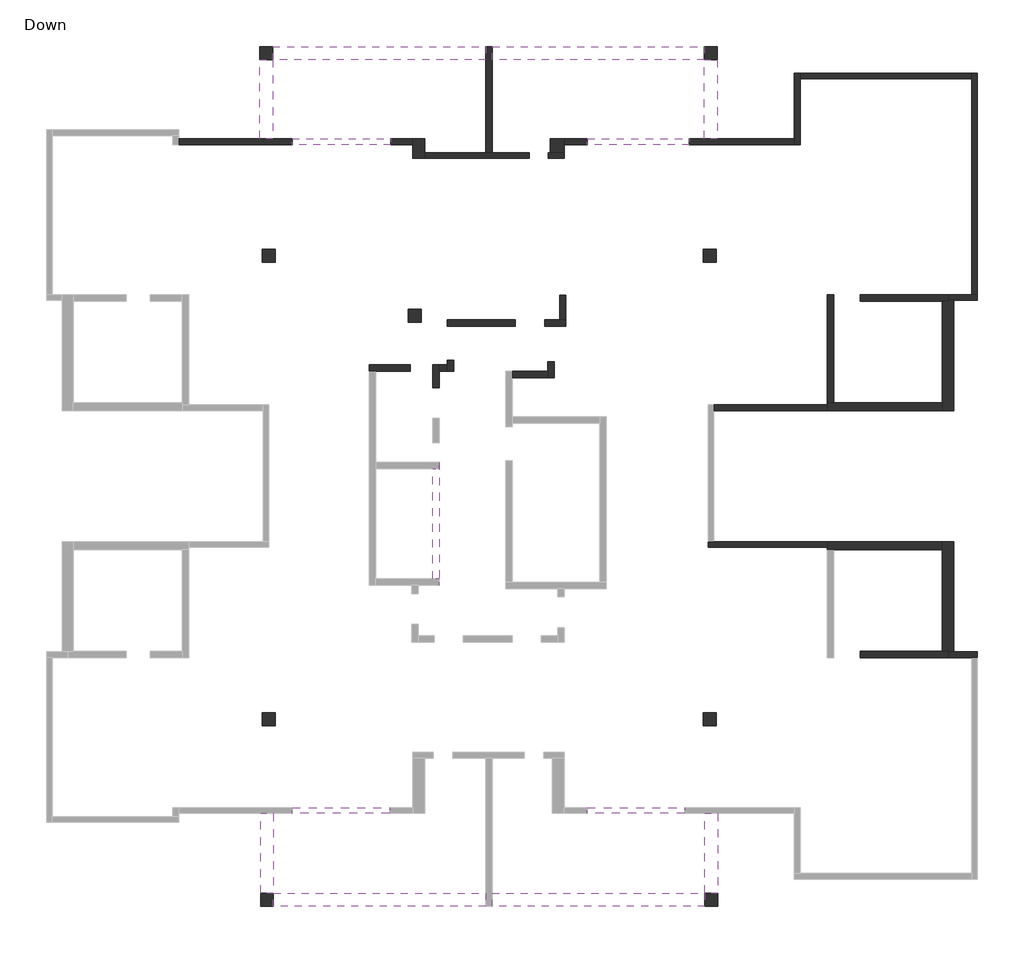
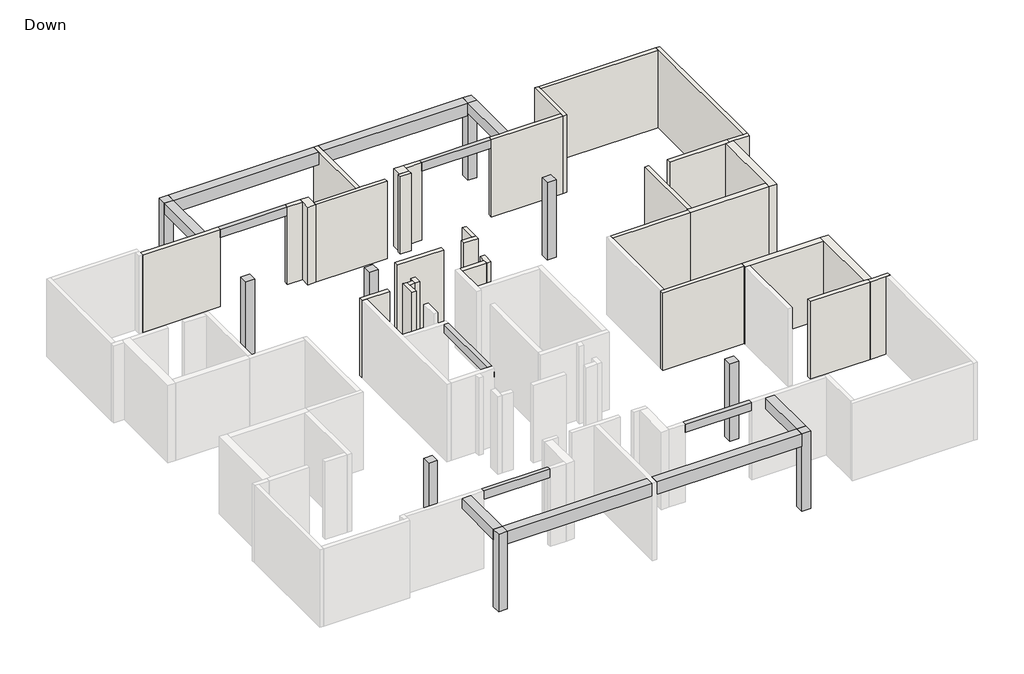
# One storey, part 2 of 2: 32 walls, 13 beams, 9 columns.
"""IFC4 building model written with IfcOpenShell, lengths in millimetres."""

from ifc_helpers import new_model, si_unit, origin, origin_with_axes, place, context, project, spatial, polyline, outline, extrude, faceted_brep, element, save

model = new_model("IFC4")

# Units and contexts
model_context = context("Model", 3, world=origin())
ifc_project = project(units=[si_unit("LENGTHUNIT", "METRE", prefix="MILLI")], contexts=[model_context])

# Site, building, storey
site = spatial("IfcSite", under=ifc_project)
building = spatial("IfcBuilding", under=site)
storey = spatial("IfcBuildingStorey", under=building, Name="Down", Elevation=0.0)

# Beams
placement = place(None, origin())
element("IfcBeam", 1, ObjectType="Concrete Rectengular Beam : 18/40", at=placement, inside=storey, context=model_context, shape_type="Brep", body=[
    faceted_brep([(-17031.2403988, 23917.8919264, 3700.0), (-17031.2403988, 23737.8919264, 3700.0), (-17031.2403988, 23737.8919264, 3540.0), (-17031.2403988, 23737.8919264, 3300.0), (-17031.2403988, 23917.8919264, 3300.0), (-17031.2403988, 23917.8919264, 3540.0), (-20181.0054246, 23917.8919264, 3300.0), (-20181.0054246, 23737.8919264, 3300.0), (-20181.0054246, 23737.8919264, 3540.0), (-20181.0054246, 23737.8919264, 3700.0), (-20181.0054246, 23917.8919264, 3700.0), (-20181.0054246, 23917.8919264, 3540.0)], [[[0, 1, 2, 3, 4, 5]], [[6, 7, 8, 9, 10, 11]], [[1, 0, 10, 9]], [[1, 9, 8, 7, 3, 2]], [[4, 3, 7, 6]], [[10, 0, 5, 4, 6, 11]]]),
])
element("IfcBeam", 2, ObjectType="Concrete Rectengular Beam : 18/40", at=placement, inside=storey, context=model_context, shape_type="Brep", body=[
    faceted_brep([(-29280.7432632, 23917.9715458, 3300.0), (-29280.7432632, 23737.9715458, 3300.0), (-29280.7432632, 23737.9715458, 3540.0), (-29280.7432632, 23737.9715458, 3700.0), (-29280.7432632, 23917.9715458, 3700.0), (-29280.7432632, 23917.9715458, 3540.0), (-26241.1471859, 23737.9715458, 3700.0), (-26241.1471859, 23917.9715458, 3700.0), (-26241.1471859, 23737.9715458, 3300.0), (-26241.1471859, 23917.9715458, 3300.0)], [[[0, 1, 2, 3, 4, 5]], [[4, 3, 6, 7]], [[2, 1, 8, 6, 3]], [[1, 0, 9, 8]], [[5, 4, 7, 9, 0]], [[7, 6, 8, 9]]]),
])
element("IfcBeam", 3, ObjectType="Concrete Rectengular Beam : 18/40", at=placement, inside=storey, context=model_context, shape_type="Brep", body=[
    faceted_brep([(-26281.3646827, 3296.899597, 3700.0), (-26281.3646827, 3116.899597, 3700.0), (-26281.3646827, 3116.899597, 3540.0), (-26281.3646827, 3116.899597, 3300.0), (-26281.3646827, 3296.899597, 3300.0), (-26281.3646827, 3296.899597, 3540.0), (-29280.7432632, 3296.899597, 3300.0), (-29280.7432632, 3116.899597, 3300.0), (-29280.7432632, 3116.899597, 3540.0), (-29280.7432632, 3116.899597, 3700.0), (-29280.7432632, 3296.899597, 3700.0), (-29280.7432632, 3296.899597, 3540.0)], [[[0, 1, 2, 3, 4, 5]], [[6, 7, 8, 9, 10, 11]], [[1, 0, 10, 9]], [[1, 9, 8, 7, 3, 2]], [[4, 3, 7, 6]], [[10, 0, 5, 4, 6, 11]]]),
])
element("IfcBeam", 4, ObjectType="Concrete Rectengular Beam : 18/40", at=placement, inside=storey, context=model_context, shape_type="Brep", body=[
    faceted_brep([(-17179.5101337, 3296.899597, 3700.0), (-17179.5101337, 3116.899597, 3700.0), (-17179.5101337, 3116.899597, 3540.0), (-17179.5101337, 3116.899597, 3300.0), (-17179.5101337, 3296.899597, 3300.0), (-17179.5101337, 3296.899597, 3540.0), (-20181.0054246, 3296.899597, 3300.0), (-20181.0054246, 3116.899597, 3300.0), (-20181.0054246, 3116.899597, 3540.0), (-20181.0054246, 3116.899597, 3700.0), (-20181.0054246, 3296.899597, 3700.0), (-20181.0054246, 3296.899597, 3540.0)], [[[0, 1, 2, 3, 4, 5]], [[6, 7, 8, 9, 10, 11]], [[1, 0, 10, 9]], [[1, 9, 8, 7, 3, 2]], [[4, 3, 7, 6]], [[10, 0, 5, 4, 6, 11]]]),
])
element("IfcBeam", 5, ObjectType="Concrete Rectengular Beam : 20/40", at=placement, inside=storey, context=model_context, shape_type="Brep", body=[
    faceted_brep([(-24949.9538662, 10346.5743227, 3700.0), (-24750.9830923, 10346.5743227, 3700.0), (-24750.9830923, 13748.1861297, 3700.0), (-24949.9538662, 13748.1861297, 3700.0), (-24949.9538662, 10346.5743227, 3300.0), (-24949.9538662, 13748.1861297, 3300.0), (-24749.9538662, 13948.1861297, 3300.0), (-24749.9538662, 10146.5743227, 3300.0), (-24750.9830923, 10146.5743227, 3300.0), (-24750.9830923, 10346.5743227, 3300.0), (-24750.9830923, 13748.1861297, 3300.0), (-24750.9830923, 13948.1861297, 3300.0), (-24749.9538662, 13948.1861297, 3540.0), (-24749.9538662, 10146.5743227, 3540.0), (-24750.9830923, 10146.5743227, 3540.0), (-24750.9830923, 13948.1861297, 3540.0), (-24750.9830923, 13748.1861297, 3540.0), (-24750.9830923, 10346.5743227, 3540.0)], [[[0, 1, 2, 3]], [[4, 0, 3, 5]], [[6, 7, 8, 9, 4, 5, 10, 11]], [[7, 6, 12, 13]], [[7, 13, 14, 8]], [[12, 6, 11, 15]], [[13, 12, 15, 16, 17, 14]], [[9, 17, 1, 0, 4]], [[17, 9, 8, 14]], [[16, 10, 5, 3, 2]], [[10, 16, 15, 11]], [[1, 17, 16, 2]]]),
])
element("IfcBeam", 6, ObjectType="Concrete Rectengular Beam : 40/50", at=placement, inside=storey, context=model_context, shape_type="Brep", body=[
    faceted_brep([(-29879.8305532, 26366.9840713, 3700.0), (-30279.8305532, 26366.9840713, 3700.0), (-30279.8305532, 23917.9715458, 3700.0), (-29879.8305532, 23917.9715458, 3700.0), (-29879.8305532, 26366.9840713, 3200.0), (-29879.8305532, 26366.9840713, 3540.0), (-29879.8305532, 23917.9715458, 3540.0), (-29879.8305532, 23917.9715458, 3200.0), (-30279.8305532, 26366.9840713, 3200.0), (-30279.8305532, 23917.9715458, 3200.0)], [[[0, 1, 2, 3]], [[4, 5, 0, 3, 6, 7]], [[8, 4, 7, 9]], [[1, 8, 9, 2]], [[1, 0, 5, 4, 8]], [[3, 2, 9, 7, 6]]]),
])
element("IfcBeam", 7, ObjectType="Concrete Rectengular Beam : 40/50", at=placement, inside=storey, context=model_context, shape_type="Brep", body=[
    faceted_brep([(-16180.4228437, 26366.9840713, 3700.0), (-16580.4228437, 26366.9840713, 3700.0), (-16580.4228437, 23917.8919264, 3700.0), (-16180.4228437, 23917.8919264, 3700.0), (-16180.4228437, 26366.9840713, 3200.0), (-16180.4228437, 23917.8919264, 3200.0), (-16580.4228437, 26366.9840713, 3200.0), (-16580.4228437, 23917.8919264, 3200.0), (-16580.4228437, 26366.9840713, 3540.0), (-16580.4228437, 23917.8919264, 3540.0)], [[[0, 1, 2, 3]], [[4, 0, 3, 5]], [[6, 4, 5, 7]], [[1, 8, 6, 7, 9, 2]], [[1, 0, 4, 6, 8]], [[3, 2, 9, 7, 5]]]),
])
element("IfcBeam", 8, ObjectType="Concrete Rectengular Beam : 40/50", at=placement, inside=storey, context=model_context, shape_type="Brep", body=[
    faceted_brep([(-30261.4923547, 659.7166846, 3700.0), (-29861.4923547, 659.7166846, 3700.0), (-29861.4923547, 3116.899597, 3700.0), (-30261.4923547, 3116.899597, 3700.0), (-29861.4923547, 659.7166846, 3540.0), (-29861.4923547, 659.7166846, 3200.0), (-29861.4923547, 3116.899597, 3200.0), (-29861.4923547, 3116.899597, 3540.0), (-30261.4923547, 659.7166846, 3200.0), (-30261.4923547, 3116.899597, 3200.0)], [[[0, 1, 2, 3]], [[1, 4, 5, 6, 7, 2]], [[5, 8, 9, 6]], [[8, 0, 3, 9]], [[5, 4, 1, 0, 8]], [[3, 2, 7, 6, 9]]]),
])
element("IfcBeam", 9, ObjectType="Concrete Rectengular Beam : 40/50", at=placement, inside=storey, context=model_context, shape_type="Brep", body=[
    faceted_brep([(-16561.2977307, 659.7166846, 3700.0), (-16161.2977307, 659.7166846, 3700.0), (-16161.2977307, 3116.899597, 3700.0), (-16561.2977307, 3116.899597, 3700.0), (-16561.2977307, 659.7166846, 3200.0), (-16561.2977307, 659.7166846, 3540.0), (-16561.2977307, 3116.899597, 3540.0), (-16561.2977307, 3116.899597, 3200.0), (-16161.2977307, 659.7166846, 3200.0), (-16161.2977307, 3116.899597, 3200.0)], [[[0, 1, 2, 3]], [[4, 5, 0, 3, 6, 7]], [[8, 4, 7, 9]], [[1, 8, 9, 2]], [[0, 5, 4, 8, 1]], [[3, 2, 9, 7, 6]]]),
])
element("IfcBeam", 10, ObjectType="Concrete Rectengular Beam : 40/60", at=placement, inside=storey, context=model_context, shape_type="Brep", body=[
    faceted_brep([(-29879.8305532, 26766.9840713, 3700.0), (-29879.8305532, 26366.9840713, 3700.0), (-23307.4000343, 26366.9840713, 3700.0), (-23307.4000343, 26766.9840713, 3700.0), (-29879.8305532, 26366.9840713, 3540.0), (-29879.8305532, 26366.9840713, 3100.0), (-23307.4000343, 26366.9840713, 3100.0), (-23307.4000343, 26366.9840713, 3540.0), (-29879.8305532, 26766.9840713, 3100.0), (-23307.4000343, 26766.9840713, 3100.0)], [[[0, 1, 2, 3]], [[1, 4, 5, 6, 7, 2]], [[5, 8, 9, 6]], [[8, 0, 3, 9]], [[1, 0, 8, 5, 4]], [[3, 2, 7, 6, 9]]]),
])
element("IfcBeam", 11, ObjectType="Concrete Rectengular Beam : 40/60", at=placement, inside=storey, context=model_context, shape_type="Brep", body=[
    faceted_brep([(-23107.4000343, 26766.9840713, 3700.0), (-23107.4000343, 26366.9840713, 3700.0), (-16580.4228437, 26366.9840713, 3700.0), (-16580.4228437, 26766.9840713, 3700.0), (-23107.4000343, 26366.9840713, 3540.0), (-23107.4000343, 26366.9840713, 3100.0), (-16580.4228437, 26366.9840713, 3100.0), (-16580.4228437, 26366.9840713, 3540.0), (-23107.4000343, 26766.9840713, 3100.0), (-16580.4228437, 26766.9840713, 3100.0)], [[[0, 1, 2, 3]], [[1, 4, 5, 6, 7, 2]], [[5, 8, 9, 6]], [[8, 0, 3, 9]], [[1, 0, 8, 5, 4]], [[3, 2, 7, 6, 9]]]),
])
element("IfcBeam", 12, ObjectType="Concrete Rectengular Beam : 40/60", at=placement, inside=storey, context=model_context, shape_type="Brep", body=[
    faceted_brep([(-29861.4923547, 659.7166846, 3700.0), (-29861.4923547, 259.7166846, 3700.0), (-23311.6200473, 259.7166846, 3700.0), (-23311.6200473, 659.7166846, 3700.0), (-29861.4923547, 259.7166846, 3100.0), (-23311.6200473, 259.7166846, 3100.0), (-29861.4923547, 659.7166846, 3100.0), (-23311.6200473, 659.7166846, 3100.0), (-29861.4923547, 659.7166846, 3540.0), (-23311.6200473, 659.7166846, 3540.0)], [[[0, 1, 2, 3]], [[1, 4, 5, 2]], [[4, 6, 7, 5]], [[6, 8, 0, 3, 9, 7]], [[1, 0, 8, 6, 4]], [[3, 2, 5, 7, 9]]]),
])
element("IfcBeam", 13, ObjectType="Concrete Rectengular Beam : 40/60", at=placement, inside=storey, context=model_context, shape_type="Brep", body=[
    faceted_brep([(-16561.2977307, 259.7166846, 3700.0), (-16561.2977307, 659.7166846, 3700.0), (-23111.6200473, 659.7166846, 3700.0), (-23111.6200473, 259.7166846, 3700.0), (-16561.2977307, 259.7166846, 3100.0), (-23111.6200473, 259.7166846, 3100.0), (-16561.2977307, 659.7166846, 3100.0), (-23111.6200473, 659.7166846, 3100.0), (-16561.2977307, 659.7166846, 3540.0), (-23111.6200473, 659.7166846, 3540.0)], [[[0, 1, 2, 3]], [[4, 0, 3, 5]], [[6, 4, 5, 7]], [[1, 8, 6, 7, 9, 2]], [[1, 0, 4, 6, 8]], [[3, 2, 9, 7, 5]]]),
])

# Columns
element("IfcColumn", 14, ObjectType="Concrete Rectengular Column : 40/40", at=placement, inside=storey, context=model_context, shape_type="Brep", body=[
    faceted_brep([(-16205.9170786, 20509.605542, 0.0), (-16205.9170786, 20109.605542, 0.0), (-16605.9170786, 20109.605542, 0.0), (-16605.9170786, 20509.605542, 0.0), (-16205.9170786, 20509.605542, 3700.0), (-16205.9170786, 20109.605542, 3700.0), (-16205.9170786, 20109.605542, 3540.0), (-16205.9170786, 20509.605542, 3540.0), (-16605.9170786, 20109.605542, 3700.0), (-16605.9170786, 20109.605542, 3540.0), (-16605.9170786, 20509.605542, 3700.0), (-16605.9170786, 20509.605542, 3540.0)], [[[0, 1, 2, 3]], [[4, 5, 6, 1, 0, 7]], [[5, 8, 9, 2, 1, 6]], [[8, 10, 11, 3, 2, 9]], [[10, 4, 7, 0, 3, 11]], [[4, 10, 8, 5]]]),
])
element("IfcColumn", 15, ObjectType="Concrete Rectengular Column : 40/40", at=placement, inside=storey, context=model_context, shape_type="Brep", body=[
    faceted_brep([(-29812.3773034, 20509.605542, 0.0), (-29812.3773034, 20109.605542, 0.0), (-30212.3773034, 20109.605542, 0.0), (-30212.3773034, 20509.605542, 0.0), (-29812.3773034, 20509.605542, 3700.0), (-29812.3773034, 20109.605542, 3700.0), (-29812.3773034, 20109.605542, 3540.0), (-29812.3773034, 20509.605542, 3540.0), (-30212.3773034, 20109.605542, 3700.0), (-30212.3773034, 20109.605542, 3540.0), (-30212.3773034, 20509.605542, 3700.0), (-30212.3773034, 20509.605542, 3540.0)], [[[0, 1, 2, 3]], [[4, 5, 6, 1, 0, 7]], [[5, 8, 9, 2, 1, 6]], [[8, 10, 11, 3, 2, 9]], [[10, 4, 7, 0, 3, 11]], [[4, 10, 8, 5]]]),
])
element("IfcColumn", 16, ObjectType="Concrete Rectengular Column : 40/40", at=placement, inside=storey, context=model_context, shape_type="Brep", body=[
    faceted_brep([(-29812.3773034, 6215.7849257, 0.0), (-29812.3773034, 5815.7849257, 0.0), (-30212.3773034, 5815.7849257, 0.0), (-30212.3773034, 6215.7849257, 0.0), (-29812.3773034, 6215.7849257, 3700.0), (-29812.3773034, 5815.7849257, 3700.0), (-29812.3773034, 5815.7849257, 3540.0), (-29812.3773034, 6215.7849257, 3540.0), (-30212.3773034, 5815.7849257, 3700.0), (-30212.3773034, 5815.7849257, 3540.0), (-30212.3773034, 6215.7849257, 3700.0), (-30212.3773034, 6215.7849257, 3540.0)], [[[0, 1, 2, 3]], [[4, 5, 6, 1, 0, 7]], [[5, 8, 9, 2, 1, 6]], [[8, 10, 11, 3, 2, 9]], [[10, 4, 7, 0, 3, 11]], [[4, 10, 8, 5]]]),
])
element("IfcColumn", 17, ObjectType="Concrete Rectengular Column : 40/40", at=placement, inside=storey, context=model_context, shape_type="Brep", body=[
    faceted_brep([(-16205.9170786, 6215.8431838, 0.0), (-16205.9170786, 5815.8431838, 0.0), (-16605.9170786, 5815.8431838, 0.0), (-16605.9170786, 6215.8431838, 0.0), (-16205.9170786, 6215.8431838, 3700.0), (-16205.9170786, 5815.8431838, 3700.0), (-16205.9170786, 5815.8431838, 3540.0), (-16205.9170786, 6215.8431838, 3540.0), (-16605.9170786, 5815.8431838, 3700.0), (-16605.9170786, 5815.8431838, 3540.0), (-16605.9170786, 6215.8431838, 3700.0), (-16605.9170786, 6215.8431838, 3540.0)], [[[0, 1, 2, 3]], [[4, 5, 6, 1, 0, 7]], [[5, 8, 9, 2, 1, 6]], [[8, 10, 11, 3, 2, 9]], [[10, 4, 7, 0, 3, 11]], [[4, 10, 8, 5]]]),
])
element("IfcColumn", 18, ObjectType="Concrete Rectengular Column : 40/40", at=placement, inside=storey, context=model_context, shape_type="Brep", body=[
    faceted_brep([(-16180.4228437, 26766.9840713, 0.0), (-16180.4228437, 26366.9840713, 0.0), (-16580.4228437, 26366.9840713, 0.0), (-16580.4228437, 26766.9840713, 0.0), (-16180.4228437, 26766.9840713, 3700.0), (-16180.4228437, 26366.9840713, 3700.0), (-16580.4228437, 26366.9840713, 3700.0), (-16580.4228437, 26366.9840713, 3100.0), (-16580.4228437, 26766.9840713, 3700.0), (-16580.4228437, 26766.9840713, 3100.0)], [[[0, 1, 2, 3]], [[4, 5, 1, 0]], [[5, 6, 7, 2, 1]], [[6, 8, 9, 3, 2, 7]], [[8, 4, 0, 3, 9]], [[4, 8, 6, 5]]]),
])
element("IfcColumn", 19, ObjectType="Concrete Rectengular Column : 40/40", at=placement, inside=storey, context=model_context, shape_type="Brep", body=[
    faceted_brep([(-29879.8305532, 26766.9840713, 0.0), (-29879.8305532, 26366.9840713, 0.0), (-30279.8305532, 26366.9840713, 0.0), (-30279.8305532, 26766.9840713, 0.0), (-29879.8305532, 26766.9840713, 3700.0), (-29879.8305532, 26366.9840713, 3700.0), (-29879.8305532, 26366.9840713, 3100.0), (-29879.8305532, 26766.9840713, 3100.0), (-30279.8305532, 26366.9840713, 3700.0), (-30279.8305532, 26766.9840713, 3700.0)], [[[0, 1, 2, 3]], [[4, 5, 6, 1, 0, 7]], [[5, 8, 2, 1, 6]], [[8, 9, 3, 2]], [[9, 4, 7, 0, 3]], [[4, 9, 8, 5]]]),
])
element("IfcColumn", 20, ObjectType="Concrete Rectengular Column : 40/40", at=placement, inside=storey, context=model_context, shape_type="SweptSolid", body=[
    extrude(outline(polyline([(-29861.4923547, 659.7166846), (-29861.4923547, 259.7166846), (-30261.4923547, 259.7166846), (-30261.4923547, 659.7166846), (-29861.4923547, 659.7166846)])), origin_with_axes(), (0.0, 0.0, 1.0), 3700.0),
])
element("IfcColumn", 21, ObjectType="Concrete Rectengular Column : 40/40", at=placement, inside=storey, context=model_context, shape_type="SweptSolid", body=[
    extrude(outline(polyline([(-16161.2977307, 659.7166846), (-16161.2977307, 259.7166846), (-16561.2977307, 259.7166846), (-16561.2977307, 659.7166846), (-16161.2977307, 659.7166846)])), origin_with_axes(), (0.0, 0.0, 1.0), 3700.0),
])
element("IfcColumn", 22, ObjectType="Concrete Rectengular Column : 40/40", at=placement, inside=storey, context=model_context, shape_type="Brep", body=[
    faceted_brep([(-25309.8528855, 18668.3919749, 0.0), (-25309.8528855, 18268.3919749, 0.0), (-25709.8528855, 18268.3919749, 0.0), (-25709.8528855, 18668.3919749, 0.0), (-25309.8528855, 18668.3919749, 3700.0), (-25309.8528855, 18268.3919749, 3700.0), (-25309.8528855, 18268.3919749, 3540.0), (-25309.8528855, 18668.3919749, 3540.0), (-25709.8528855, 18268.3919749, 3700.0), (-25709.8528855, 18268.3919749, 3540.0), (-25709.8528855, 18668.3919749, 3700.0), (-25709.8528855, 18668.3919749, 3540.0)], [[[0, 1, 2, 3]], [[4, 5, 6, 1, 0, 7]], [[5, 8, 9, 2, 1, 6]], [[8, 10, 11, 3, 2, 9]], [[10, 4, 7, 0, 3, 11]], [[4, 10, 8, 5]]]),
])

# Walls
element("IfcWall", 23, ObjectType="18", at=placement, inside=storey, context=model_context, shape_type="Brep", body=[
    faceted_brep([(-8149.623737, 8097.598694, 0.0), (-8879.8888113, 8097.598694, 0.0), (-9054.8888113, 8097.598694, 0.0), (-9054.8888113, 8097.598694, 3700.0), (-8879.8888113, 8097.598694, 3700.0), (-8149.623737, 8097.598694, 3700.0), (-8149.623737, 7917.598694, 0.0), (-8149.623737, 7917.598694, 3700.0), (-8329.623737, 7917.598694, 3700.0), (-9054.8888113, 7917.598694, 3700.0), (-9054.8888113, 7917.598694, 3540.0), (-9054.8888113, 7917.598694, 0.0), (-8329.623737, 7917.598694, 0.0)], [[[0, 1, 2, 3, 4, 5]], [[6, 7, 8, 9, 10, 11, 12]], [[2, 1, 0, 6, 12, 11]], [[3, 2, 11, 10, 9]], [[5, 4, 3, 9, 8, 7]], [[0, 5, 7, 6]]]),
])
element("IfcWall", 24, ObjectType="18", at=placement, inside=storey, context=model_context, shape_type="Brep", body=[
    faceted_brep([(-12779.898521, 11497.0355326, 0.0), (-16279.8286113, 11497.0355326, 0.0), (-16459.8286113, 11497.0355326, 0.0), (-16459.8286113, 11497.0355326, 3700.0), (-16279.8286113, 11497.0355326, 3700.0), (-12779.898521, 11497.0355326, 3700.0), (-12779.898521, 11317.0355326, 0.0), (-12779.898521, 11317.0355326, 3540.0), (-12779.898521, 11317.0355326, 3700.0), (-16459.8286113, 11317.0355326, 3700.0), (-16459.8286113, 11317.0355326, 3540.0), (-16459.8286113, 11317.0355326, 0.0)], [[[0, 1, 2, 3, 4, 5]], [[6, 7, 8, 9, 10, 11]], [[2, 1, 0, 6, 11]], [[5, 4, 3, 9, 8]], [[0, 5, 8, 7, 6]], [[3, 2, 11, 10, 9]]]),
])
element("IfcWall", 25, ObjectType="18", at=placement, inside=storey, context=model_context, shape_type="Brep", body=[
    faceted_brep([(-32781.782199, 23737.9715458, 0.0), (-29280.7432632, 23737.9715458, 0.0), (-29280.7432632, 23737.9715458, 3300.0), (-29280.7432632, 23737.9715458, 3700.0), (-32781.782199, 23737.9715458, 3700.0), (-32781.782199, 23917.9715458, 0.0), (-32781.782199, 23917.9715458, 3700.0), (-30279.8305532, 23917.9715458, 3700.0), (-29879.8305532, 23917.9715458, 3700.0), (-29280.7432632, 23917.9715458, 3700.0), (-29280.7432632, 23917.9715458, 3300.0), (-29280.7432632, 23917.9715458, 0.0)], [[[0, 1, 2, 3, 4]], [[5, 6, 7, 8, 9, 10, 11]], [[1, 0, 5, 11]], [[3, 2, 1, 11, 10, 9]], [[4, 3, 9, 8, 7, 6]], [[0, 4, 6, 5]]]),
])
element("IfcWall", 26, ObjectType="18", at=placement, inside=storey, context=model_context, shape_type="Brep", body=[
    faceted_brep([(-25199.7256887, 23316.7461841, 0.0), (-21979.7256887, 23316.7461841, 0.0), (-21979.7256887, 23316.7461841, 3700.0), (-25199.7256887, 23316.7461841, 3700.0), (-25199.7256887, 23496.7461841, 0.0), (-25199.7256887, 23496.7461841, 3540.0), (-25199.7256887, 23496.7461841, 3700.0), (-23307.4000343, 23496.7461841, 3700.0), (-23107.4000343, 23496.7461841, 3700.0), (-21979.7256887, 23496.7461841, 3700.0), (-21979.7256887, 23496.7461841, 3540.0), (-21979.7256887, 23496.7461841, 0.0), (-23107.4000343, 23496.7461841, 0.0), (-23307.4000343, 23496.7461841, 0.0)], [[[0, 1, 2, 3]], [[4, 5, 6, 7, 8, 9, 10, 11, 12, 13]], [[1, 0, 4, 13, 12, 11]], [[2, 1, 11, 10, 9]], [[3, 2, 9, 8, 7, 6]], [[0, 3, 6, 5, 4]]]),
])
element("IfcWall", 27, ObjectType="18", at=placement, inside=storey, context=model_context, shape_type="Brep", body=[
    faceted_brep([(-8149.623737, 19117.1928294, 0.0), (-8149.623737, 25947.8171618, 0.0), (-8149.623737, 25947.8171618, 3700.0), (-8149.623737, 19117.1928294, 3700.0), (-8329.623737, 19117.1928294, 0.0), (-8329.623737, 19117.1928294, 3540.0), (-8329.623737, 19117.1928294, 3700.0), (-8329.623737, 25767.8171618, 3700.0), (-8329.623737, 25947.8171618, 3700.0), (-8329.623737, 25947.8171618, 0.0), (-8329.623737, 25767.8171618, 0.0)], [[[0, 1, 2, 3]], [[4, 5, 6, 7, 8, 9, 10]], [[1, 0, 4, 10, 9]], [[3, 2, 8, 7, 6]], [[0, 3, 6, 5, 4]], [[2, 1, 9, 8]]]),
])
element("IfcWall", 28, ObjectType="18", at=placement, inside=storey, context=model_context, shape_type="Brep", body=[
    faceted_brep([(-13801.2403988, 25947.8171618, 0.0), (-13801.2403988, 23917.8919264, 0.0), (-13801.2403988, 23737.8919264, 0.0), (-13801.2403988, 23737.8919264, 3700.0), (-13801.2403988, 23917.8919264, 3700.0), (-13801.2403988, 25947.8171618, 3700.0), (-13621.2403988, 25947.8171618, 0.0), (-13621.2403988, 25947.8171618, 3700.0), (-13621.2403988, 25767.8171618, 3700.0), (-13621.2403988, 23737.8919264, 3700.0), (-13621.2403988, 23737.8919264, 3540.0), (-13621.2403988, 23737.8919264, 0.0), (-13621.2403988, 25767.8171618, 0.0)], [[[0, 1, 2, 3, 4, 5]], [[6, 7, 8, 9, 10, 11, 12]], [[2, 1, 0, 6, 12, 11]], [[5, 4, 3, 9, 8, 7]], [[3, 2, 11, 10, 9]], [[0, 5, 7, 6]]]),
])
element("IfcWall", 29, ObjectType="18", at=placement, inside=storey, context=model_context, shape_type="Brep", body=[
    faceted_brep([(-13801.2403988, 23917.8919264, 0.0), (-17031.2403988, 23917.8919264, 0.0), (-17031.2403988, 23917.8919264, 3300.0), (-17031.2403988, 23917.8919264, 3700.0), (-16580.4228437, 23917.8919264, 3700.0), (-16180.4228437, 23917.8919264, 3700.0), (-13801.2403988, 23917.8919264, 3700.0), (-13801.2403988, 23737.8919264, 0.0), (-13801.2403988, 23737.8919264, 3700.0), (-17031.2403988, 23737.8919264, 3700.0), (-17031.2403988, 23737.8919264, 3300.0), (-17031.2403988, 23737.8919264, 0.0)], [[[0, 1, 2, 3, 4, 5, 6]], [[7, 8, 9, 10, 11]], [[1, 0, 7, 11]], [[3, 2, 1, 11, 10, 9]], [[6, 5, 4, 3, 9, 8]], [[0, 6, 8, 7]]]),
])
element("IfcWall", 30, ObjectType="18", at=placement, inside=storey, context=model_context, shape_type="Brep", body=[
    faceted_brep([(-8149.623737, 19117.1928294, 0.0), (-8329.623737, 19117.1928294, 0.0), (-9054.8888113, 19117.1928294, 0.0), (-9054.8888113, 19117.1928294, 3540.0), (-9054.8888113, 19117.1928294, 3700.0), (-8329.623737, 19117.1928294, 3700.0), (-8149.623737, 19117.1928294, 3700.0), (-8149.623737, 18937.1928294, 0.0), (-8149.623737, 18937.1928294, 3700.0), (-8879.8888113, 18937.1928294, 3700.0), (-9054.8888113, 18937.1928294, 3700.0), (-9054.8888113, 18937.1928294, 0.0), (-8879.8888113, 18937.1928294, 0.0)], [[[0, 1, 2, 3, 4, 5, 6]], [[7, 8, 9, 10, 11, 12]], [[2, 1, 0, 7, 12, 11]], [[4, 3, 2, 11, 10]], [[6, 5, 4, 10, 9, 8]], [[0, 6, 8, 7]]]),
])
element("IfcWall", 31, ObjectType="18", at=placement, inside=storey, context=model_context, shape_type="Brep", body=[
    faceted_brep([(-12779.898521, 15717.7559909, 0.0), (-16279.8286113, 15717.7559909, 0.0), (-16279.8286113, 15717.7559909, 3700.0), (-12779.898521, 15717.7559909, 3700.0), (-12779.898521, 15717.7559909, 3540.0), (-12779.898521, 15537.7559909, 0.0), (-12779.898521, 15537.7559909, 3700.0), (-16279.8286113, 15537.7559909, 3700.0), (-16279.8286113, 15537.7559909, 0.0)], [[[0, 1, 2, 3, 4]], [[5, 6, 7, 8]], [[1, 0, 5, 8]], [[3, 2, 7, 6]], [[0, 4, 3, 6, 5]], [[2, 1, 8, 7]]]),
])
element("IfcWall", 32, ObjectType="18", at=placement, inside=storey, context=model_context, shape_type="Brep", body=[
    faceted_brep([(-8329.623737, 25947.8171618, 0.0), (-13621.2403988, 25947.8171618, 0.0), (-13621.2403988, 25947.8171618, 3700.0), (-8329.623737, 25947.8171618, 3700.0), (-8329.623737, 25767.8171618, 0.0), (-8329.623737, 25767.8171618, 3540.0), (-8329.623737, 25767.8171618, 3700.0), (-13621.2403988, 25767.8171618, 3700.0), (-13621.2403988, 25767.8171618, 3540.0), (-13621.2403988, 25767.8171618, 0.0)], [[[0, 1, 2, 3]], [[4, 5, 6, 7, 8, 9]], [[1, 0, 4, 9]], [[3, 2, 7, 6]], [[0, 3, 6, 5, 4]], [[2, 1, 9, 8, 7]]]),
])
element("IfcWall", 33, ObjectType="18", at=placement, inside=storey, context=model_context, shape_type="Brep", body=[
    faceted_brep([(-25559.7256887, 23917.8919264, 0.0), (-26241.1471859, 23917.8919264, 0.0), (-26241.1471859, 23917.8919264, 3700.0), (-25559.7256887, 23917.8919264, 3700.0), (-25559.7256887, 23737.8919264, 0.0), (-25559.7256887, 23737.8919264, 3540.0), (-25559.7256887, 23737.8919264, 3700.0), (-26241.1471859, 23737.8919264, 3700.0), (-26241.1471859, 23737.8919264, 0.0)], [[[0, 1, 2, 3]], [[4, 5, 6, 7, 8]], [[1, 0, 4, 8]], [[2, 1, 8, 7]], [[3, 2, 7, 6]], [[0, 3, 6, 5, 4]]]),
])
element("IfcWall", 34, ObjectType="18", at=placement, inside=storey, context=model_context, shape_type="Brep", body=[
    faceted_brep([(-21381.1801988, 23316.7461841, 0.0), (-20900.686947, 23316.7461841, 0.0), (-20900.686947, 23316.7461841, 3540.0), (-20900.686947, 23316.7461841, 3700.0), (-21381.1801988, 23316.7461841, 3700.0), (-21381.1801988, 23496.7461841, 0.0), (-21381.1801988, 23496.7461841, 3540.0), (-21381.1801988, 23496.7461841, 3700.0), (-21330.686947, 23496.7461841, 3700.0), (-20900.686947, 23496.7461841, 3700.0), (-20900.686947, 23496.7461841, 0.0), (-21330.686947, 23496.7461841, 0.0)], [[[0, 1, 2, 3, 4]], [[5, 6, 7, 8, 9, 10, 11]], [[1, 0, 5, 11, 10]], [[4, 3, 9, 8, 7]], [[0, 4, 7, 6, 5]], [[3, 2, 1, 10, 9]]]),
])
element("IfcWall", 35, ObjectType="18", at=placement, inside=storey, context=model_context, shape_type="Brep", body=[
    faceted_brep([(-20900.686947, 23737.8919264, 0.0), (-20181.0054246, 23737.8919264, 0.0), (-20181.0054246, 23737.8919264, 3300.0), (-20181.0054246, 23737.8919264, 3700.0), (-20900.686947, 23737.8919264, 3700.0), (-20900.686947, 23737.8919264, 3540.0), (-20900.686947, 23917.8919264, 0.0), (-20900.686947, 23917.8919264, 3700.0), (-20181.0054246, 23917.8919264, 3700.0), (-20181.0054246, 23917.8919264, 3300.0), (-20181.0054246, 23917.8919264, 0.0)], [[[0, 1, 2, 3, 4, 5]], [[6, 7, 8, 9, 10]], [[1, 0, 6, 10]], [[3, 2, 1, 10, 9, 8]], [[4, 3, 8, 7]], [[0, 5, 4, 7, 6]]]),
])
element("IfcWall", 36, ObjectType="18", at=placement, inside=storey, context=model_context, shape_type="Brep", body=[
    faceted_brep([(-20849.8858984, 18347.7394844, 0.0), (-20849.8858984, 19098.1424361, 0.0), (-20849.8858984, 19098.1424361, 3540.0), (-20849.8858984, 19098.1424361, 3700.0), (-20849.8858984, 18347.7394844, 3700.0), (-21029.8858984, 18347.7394844, 0.0), (-21029.8858984, 18347.7394844, 3540.0), (-21029.8858984, 18347.7394844, 3700.0), (-21029.8858984, 19098.1424361, 3700.0), (-21029.8858984, 19098.1424361, 3540.0), (-21029.8858984, 19098.1424361, 0.0)], [[[0, 1, 2, 3, 4]], [[5, 6, 7, 8, 9, 10]], [[1, 0, 5, 10]], [[3, 2, 1, 10, 9, 8]], [[4, 3, 8, 7]], [[0, 4, 7, 6, 5]]]),
])
element("IfcWall", 37, ObjectType="20", at=placement, inside=storey, context=model_context, shape_type="Brep", body=[
    faceted_brep([(-11760.7316116, 7916.6490873, 0.0), (-9054.8888113, 7916.6490873, 0.0), (-9054.8888113, 7916.6490873, 3540.0), (-9054.8888113, 7916.6490873, 3700.0), (-11760.7316116, 7916.6490873, 3700.0), (-11760.7316116, 7916.6490873, 3540.0), (-11760.7316116, 8116.6490873, 0.0), (-11760.7316116, 8116.6490873, 3540.0), (-11760.7316116, 8116.6490873, 3700.0), (-9229.8888113, 8116.6490873, 3700.0), (-9054.8888113, 8116.6490873, 3700.0), (-9054.8888113, 8116.6490873, 0.0), (-9229.8888113, 8116.6490873, 0.0), (-9054.8888113, 8097.598694, 0.0), (-9054.8888113, 7917.598694, 0.0), (-9054.8888113, 8097.598694, 3700.0), (-9054.8888113, 7917.598694, 3700.0)], [[[0, 1, 2, 3, 4, 5]], [[6, 7, 8, 9, 10, 11, 12]], [[1, 0, 6, 12, 11, 13, 14]], [[3, 2, 1, 14, 13, 11, 10, 15, 16]], [[4, 3, 16, 15, 10, 9, 8]], [[0, 5, 4, 8, 7, 6]]]),
])
element("IfcWall", 38, ObjectType="20", at=placement, inside=storey, context=model_context, shape_type="Brep", body=[
    faceted_brep([(-23107.4000343, 23496.7461841, 0.0), (-23107.4000343, 26766.9840713, 0.0), (-23107.4000343, 26766.9840713, 3100.0), (-23107.4000343, 26766.9840713, 3700.0), (-23107.4000343, 26366.9840713, 3700.0), (-23107.4000343, 23496.7461841, 3700.0), (-23107.4000343, 23496.7461841, 3540.0), (-23307.4000343, 23496.7461841, 0.0), (-23307.4000343, 23496.7461841, 3540.0), (-23307.4000343, 23496.7461841, 3700.0), (-23307.4000343, 26366.9840713, 3700.0), (-23307.4000343, 26766.9840713, 3700.0), (-23307.4000343, 26766.9840713, 3100.0), (-23307.4000343, 26766.9840713, 0.0)], [[[0, 1, 2, 3, 4, 5, 6]], [[7, 8, 9, 10, 11, 12, 13]], [[1, 0, 7, 13]], [[3, 2, 1, 13, 12, 11]], [[5, 4, 3, 11, 10, 9]], [[0, 6, 5, 9, 8, 7]]]),
])
element("IfcWall", 39, ObjectType="20", at=placement, inside=storey, context=model_context, shape_type="Brep", body=[
    faceted_brep([(-11760.7316116, 18918.1424361, 0.0), (-9229.8888113, 18918.1424361, 0.0), (-9054.8888113, 18918.1424361, 0.0), (-9054.8888113, 18918.1424361, 3700.0), (-9229.8888113, 18918.1424361, 3700.0), (-11760.7316116, 18918.1424361, 3700.0), (-11760.7316116, 18918.1424361, 3540.0), (-11760.7316116, 19118.1424361, 0.0), (-11760.7316116, 19118.1424361, 3540.0), (-11760.7316116, 19118.1424361, 3700.0), (-9054.8888113, 19118.1424361, 3700.0), (-9054.8888113, 19118.1424361, 3540.0), (-9054.8888113, 19118.1424361, 0.0), (-9054.8888113, 19117.1928294, 0.0), (-9054.8888113, 18937.1928294, 0.0), (-9054.8888113, 19117.1928294, 3700.0), (-9054.8888113, 18937.1928294, 3700.0)], [[[0, 1, 2, 3, 4, 5, 6]], [[7, 8, 9, 10, 11, 12]], [[2, 1, 0, 7, 12, 13, 14]], [[3, 2, 14, 13, 12, 11, 10, 15, 16]], [[5, 4, 3, 16, 15, 10, 9]], [[0, 6, 5, 9, 8, 7]]]),
])
element("IfcWall", 40, ObjectType="20", at=placement, inside=storey, context=model_context, shape_type="Brep", body=[
    faceted_brep([(-12579.898521, 15787.7559909, 0.0), (-12579.898521, 19117.11321, 0.0), (-12579.898521, 19117.11321, 3540.0), (-12579.898521, 19117.11321, 3700.0), (-12579.898521, 18918.1424361, 3700.0), (-12579.898521, 15787.7559909, 3700.0), (-12579.898521, 15787.7559909, 3540.0), (-12779.898521, 15787.7559909, 0.0), (-12779.898521, 15787.7559909, 3700.0), (-12779.898521, 19117.11321, 3700.0), (-12779.898521, 19117.11321, 3540.0), (-12779.898521, 19117.11321, 0.0)], [[[0, 1, 2, 3, 4, 5, 6]], [[7, 8, 9, 10, 11]], [[1, 0, 7, 11]], [[3, 2, 1, 11, 10, 9]], [[5, 4, 3, 9, 8]], [[0, 6, 5, 8, 7]]]),
])
element("IfcWall", 41, ObjectType="20", at=placement, inside=storey, context=model_context, shape_type="Brep", body=[
    faceted_brep([(-22500.9199794, 16546.4772259, 0.0), (-21401.2598182, 16546.4772259, 0.0), (-21401.2598182, 16546.4772259, 3700.0), (-22500.9199794, 16546.4772259, 3700.0), (-22500.9199794, 16546.4772259, 3540.0), (-22500.9199794, 16746.4772259, 0.0), (-22500.9199794, 16746.4772259, 3700.0), (-21401.2598182, 16746.4772259, 3700.0), (-21401.2598182, 16746.4772259, 3540.0), (-21401.2598182, 16746.4772259, 0.0)], [[[0, 1, 2, 3, 4]], [[5, 6, 7, 8, 9]], [[1, 0, 5, 9]], [[3, 2, 7, 6]], [[0, 4, 3, 6, 5]], [[2, 1, 9, 8, 7]]]),
])
element("IfcWall", 42, ObjectType="20", at=placement, inside=storey, context=model_context, shape_type="Brep", body=[
    faceted_brep([(-21201.2598182, 16546.4772259, 0.0), (-21201.2598182, 17047.0500971, 0.0), (-21201.2598182, 17047.0500971, 3540.0), (-21201.2598182, 17047.0500971, 3700.0), (-21201.2598182, 16546.4772259, 3700.0), (-21201.2598182, 16546.4772259, 3540.0), (-21401.2598182, 16546.4772259, 0.0), (-21401.2598182, 16546.4772259, 3700.0), (-21401.2598182, 16746.4772259, 3700.0), (-21401.2598182, 17047.0500971, 3700.0), (-21401.2598182, 17047.0500971, 3540.0), (-21401.2598182, 17047.0500971, 0.0), (-21401.2598182, 16746.4772259, 0.0)], [[[0, 1, 2, 3, 4, 5]], [[6, 7, 8, 9, 10, 11, 12]], [[1, 0, 6, 12, 11]], [[3, 2, 1, 11, 10, 9]], [[4, 3, 9, 8, 7]], [[0, 5, 4, 7, 6]]]),
])
element("IfcWall", 43, ObjectType="20", at=placement, inside=storey, context=model_context, shape_type="Brep", body=[
    faceted_brep([(-21499.715979, 18147.7394844, 0.0), (-20849.8858984, 18147.7394844, 0.0), (-20849.8858984, 18147.7394844, 3540.0), (-20849.8858984, 18147.7394844, 3700.0), (-21499.715979, 18147.7394844, 3700.0), (-21499.715979, 18147.7394844, 3540.0), (-21499.715979, 18347.7394844, 0.0), (-21499.715979, 18347.7394844, 3540.0), (-21499.715979, 18347.7394844, 3700.0), (-21029.8858984, 18347.7394844, 3700.0), (-20849.8858984, 18347.7394844, 3700.0), (-20849.8858984, 18347.7394844, 0.0), (-21029.8858984, 18347.7394844, 0.0)], [[[0, 1, 2, 3, 4, 5]], [[6, 7, 8, 9, 10, 11, 12]], [[1, 0, 6, 12, 11]], [[4, 3, 10, 9, 8]], [[0, 5, 4, 8, 7, 6]], [[3, 2, 1, 11, 10]]]),
])
element("IfcWall", 44, ObjectType="20", at=placement, inside=storey, context=model_context, shape_type="Brep", body=[
    faceted_brep([(-22401.4345924, 18346.7102583, 0.0), (-24501.2112698, 18346.7102583, 0.0), (-24501.2112698, 18346.7102583, 3540.0), (-24501.2112698, 18346.7102583, 3700.0), (-22401.4345924, 18346.7102583, 3700.0), (-22401.4345924, 18346.7102583, 3540.0), (-22401.4345924, 18146.7102583, 0.0), (-22401.4345924, 18146.7102583, 3540.0), (-22401.4345924, 18146.7102583, 3700.0), (-24501.2112698, 18146.7102583, 3700.0), (-24501.2112698, 18146.7102583, 3540.0), (-24501.2112698, 18146.7102583, 0.0)], [[[0, 1, 2, 3, 4, 5]], [[6, 7, 8, 9, 10, 11]], [[1, 0, 6, 11]], [[3, 2, 1, 11, 10, 9]], [[4, 3, 9, 8]], [[0, 5, 4, 8, 7, 6]]]),
])
element("IfcWall", 45, ObjectType="20", at=placement, inside=storey, context=model_context, shape_type="Brep", body=[
    faceted_brep([(-24500.1237856, 17097.8511457, 0.0), (-24500.1237856, 16946.4772259, 0.0), (-24500.1237856, 16746.4772259, 0.0), (-24500.1237856, 16746.4772259, 3700.0), (-24500.1237856, 16946.4772259, 3700.0), (-24500.1237856, 17097.8511457, 3700.0), (-24500.1237856, 17097.8511457, 3540.0), (-24300.1237856, 17097.8511457, 0.0), (-24300.1237856, 17097.8511457, 3540.0), (-24300.1237856, 17097.8511457, 3700.0), (-24300.1237856, 16746.4772259, 3700.0), (-24300.1237856, 16746.4772259, 3540.0), (-24300.1237856, 16746.4772259, 0.0)], [[[0, 1, 2, 3, 4, 5, 6]], [[7, 8, 9, 10, 11, 12]], [[2, 1, 0, 7, 12]], [[5, 4, 3, 10, 9]], [[0, 6, 5, 9, 8, 7]], [[3, 2, 12, 11, 10]]]),
])
element("IfcWall", 46, ObjectType="20", at=placement, inside=storey, context=model_context, shape_type="Brep", body=[
    faceted_brep([(-24500.1237856, 16946.4772259, 0.0), (-24749.9538662, 16946.4772259, 0.0), (-24749.9538662, 16946.4772259, 3700.0), (-24500.1237856, 16946.4772259, 3700.0), (-24500.1237856, 16946.4772259, 3540.0), (-24500.1237856, 16746.4772259, 0.0), (-24500.1237856, 16746.4772259, 3700.0), (-24749.9538662, 16746.4772259, 3700.0), (-24749.9538662, 16746.4772259, 3540.0), (-24749.9538662, 16746.4772259, 0.0)], [[[0, 1, 2, 3, 4]], [[5, 6, 7, 8, 9]], [[1, 0, 5, 9]], [[3, 2, 7, 6]], [[0, 4, 3, 6, 5]], [[2, 1, 9, 8, 7]]]),
])
element("IfcWall", 47, ObjectType="20", at=placement, inside=storey, context=model_context, shape_type="Brep", body=[
    faceted_brep([(-24949.9538662, 16946.4772259, 0.0), (-24949.9538662, 16246.9335809, 0.0), (-24949.9538662, 16246.9335809, 3540.0), (-24949.9538662, 16246.9335809, 3700.0), (-24949.9538662, 16946.4772259, 3700.0), (-24949.9538662, 16946.4772259, 3540.0), (-24749.9538662, 16946.4772259, 0.0), (-24749.9538662, 16946.4772259, 3700.0), (-24749.9538662, 16746.4772259, 3700.0), (-24749.9538662, 16246.9335809, 3700.0), (-24749.9538662, 16246.9335809, 3540.0), (-24749.9538662, 16246.9335809, 0.0), (-24749.9538662, 16746.4772259, 0.0)], [[[0, 1, 2, 3, 4, 5]], [[6, 7, 8, 9, 10, 11, 12]], [[1, 0, 6, 12, 11]], [[3, 2, 1, 11, 10, 9]], [[4, 3, 9, 8, 7]], [[0, 5, 4, 7, 6]]]),
])
element("IfcWall", 48, ObjectType="20", at=placement, inside=storey, context=model_context, shape_type="Brep", body=[
    faceted_brep([(-25650.5849954, 16947.5647102, 0.0), (-26901.5608183, 16947.5647102, 0.0), (-26901.5608183, 16947.5647102, 3540.0), (-26901.5608183, 16947.5647102, 3700.0), (-25650.5849954, 16947.5647102, 3700.0), (-25650.5849954, 16947.5647102, 3540.0), (-25650.5849954, 16747.5647102, 0.0), (-25650.5849954, 16747.5647102, 3540.0), (-25650.5849954, 16747.5647102, 3700.0), (-26701.5608183, 16747.5647102, 3700.0), (-26901.5608183, 16747.5647102, 3700.0), (-26901.5608183, 16747.5647102, 0.0), (-26701.5608183, 16747.5647102, 0.0), (-25650.5849954, 16946.4772259, 3700.0)], [[[0, 1, 2, 3, 4, 5]], [[6, 7, 8, 9, 10, 11, 12]], [[1, 0, 6, 12, 11]], [[4, 3, 10, 9, 8, 13]], [[0, 5, 4, 13, 8, 7, 6]], [[3, 2, 1, 11, 10]]]),
])
element("IfcWall", 49, ObjectType="25", at=placement, inside=storey, context=model_context, shape_type="Brep", body=[
    faceted_brep([(-9229.8888113, 11497.0355326, 0.0), (-12779.898521, 11497.0355326, 0.0), (-12779.898521, 11497.0355326, 3700.0), (-9229.8888113, 11497.0355326, 3700.0), (-9229.8888113, 11247.0355326, 0.0), (-9229.8888113, 11247.0355326, 3540.0), (-9229.8888113, 11247.0355326, 3700.0), (-12579.898521, 11247.0355326, 3700.0), (-12779.898521, 11247.0355326, 3700.0), (-12779.898521, 11247.0355326, 0.0), (-12579.898521, 11247.0355326, 0.0), (-12779.898521, 11317.0355326, 0.0), (-12779.898521, 11317.0355326, 3700.0)], [[[0, 1, 2, 3]], [[4, 5, 6, 7, 8, 9, 10]], [[1, 0, 4, 10, 9, 11]], [[3, 2, 12, 8, 7, 6]], [[0, 3, 6, 5, 4]], [[2, 1, 11, 9, 8, 12]]]),
])
element("IfcWall", 50, ObjectType="25", at=placement, inside=storey, context=model_context, shape_type="Brep", body=[
    faceted_brep([(-9229.8888113, 15787.7559909, 0.0), (-12579.898521, 15787.7559909, 0.0), (-12779.898521, 15787.7559909, 0.0), (-12779.898521, 15787.7559909, 3700.0), (-12579.898521, 15787.7559909, 3700.0), (-9229.8888113, 15787.7559909, 3700.0), (-9229.8888113, 15787.7559909, 3540.0), (-9229.8888113, 15537.7559909, 0.0), (-9229.8888113, 15537.7559909, 3700.0), (-12779.898521, 15537.7559909, 3700.0), (-12779.898521, 15537.7559909, 0.0), (-12779.898521, 15717.7559909, 0.0), (-12779.898521, 15717.7559909, 3700.0)], [[[0, 1, 2, 3, 4, 5, 6]], [[7, 8, 9, 10]], [[2, 1, 0, 7, 10, 11]], [[5, 4, 3, 12, 9, 8]], [[0, 6, 5, 8, 7]], [[3, 2, 11, 10, 9, 12]]]),
])
element("IfcWall", 51, ObjectType="35", at=placement, inside=storey, context=model_context, shape_type="Brep", body=[
    faceted_brep([(-8879.8888113, 8097.598694, 0.0), (-8879.8888113, 11497.0355326, 0.0), (-8879.8888113, 11497.0355326, 3700.0), (-8879.8888113, 8097.598694, 3700.0), (-9229.8888113, 8116.6490873, 0.0), (-9229.8888113, 8116.6490873, 3540.0), (-9229.8888113, 8116.6490873, 3700.0), (-9229.8888113, 11247.0355326, 3700.0), (-9229.8888113, 11497.0355326, 3700.0), (-9229.8888113, 11497.0355326, 0.0), (-9229.8888113, 11247.0355326, 0.0), (-9054.8888113, 8097.598694, 0.0), (-9054.8888113, 8116.6490873, 0.0), (-9054.8888113, 8116.6490873, 3700.0), (-9054.8888113, 8097.598694, 3700.0)], [[[0, 1, 2, 3]], [[4, 5, 6, 7, 8, 9, 10]], [[1, 0, 11, 12, 4, 10, 9]], [[3, 2, 8, 7, 6, 13, 14]], [[0, 3, 14, 11]], [[14, 13, 12, 11]], [[13, 6, 5, 4, 12]], [[2, 1, 9, 8]]]),
])
element("IfcWall", 52, ObjectType="35", at=placement, inside=storey, context=model_context, shape_type="Brep", body=[
    faceted_brep([(-9229.8888113, 18918.1424361, 0.0), (-9229.8888113, 15787.7559909, 0.0), (-9229.8888113, 15537.7559909, 0.0), (-9229.8888113, 15537.7559909, 3700.0), (-9229.8888113, 15787.7559909, 3700.0), (-9229.8888113, 18918.1424361, 3700.0), (-9229.8888113, 18918.1424361, 3540.0), (-8879.8888113, 18937.1928294, 0.0), (-8879.8888113, 18937.1928294, 3700.0), (-8879.8888113, 15537.7559909, 3700.0), (-8879.8888113, 15537.7559909, 0.0), (-9054.8888113, 18918.1424361, 0.0), (-9054.8888113, 18937.1928294, 0.0), (-9054.8888113, 18937.1928294, 3700.0), (-9054.8888113, 18918.1424361, 3700.0)], [[[0, 1, 2, 3, 4, 5, 6]], [[7, 8, 9, 10]], [[2, 1, 0, 11, 12, 7, 10]], [[5, 4, 3, 9, 8, 13, 14]], [[0, 6, 5, 14, 11]], [[14, 13, 12, 11]], [[13, 8, 7, 12]], [[3, 2, 10, 9]]]),
])
element("IfcWall", 53, ObjectType="36", at=placement, inside=storey, context=model_context, shape_type="Brep", body=[
    faceted_brep([(-25559.7256887, 23917.8919264, 0.0), (-25559.7256887, 23737.8919264, 0.0), (-25559.7256887, 23316.7461841, 0.0), (-25559.7256887, 23316.7461841, 3540.0), (-25559.7256887, 23316.7461841, 3700.0), (-25559.7256887, 23737.8919264, 3700.0), (-25559.7256887, 23917.8919264, 3700.0), (-25199.7256887, 23917.8919264, 0.0), (-25199.7256887, 23917.8919264, 3540.0), (-25199.7256887, 23917.8919264, 3700.0), (-25199.7256887, 23496.7461841, 3700.0), (-25199.7256887, 23316.7461841, 3700.0), (-25199.7256887, 23316.7461841, 0.0), (-25199.7256887, 23496.7461841, 0.0)], [[[0, 1, 2, 3, 4, 5, 6]], [[7, 8, 9, 10, 11, 12, 13]], [[2, 1, 0, 7, 13, 12]], [[6, 5, 4, 11, 10, 9]], [[4, 3, 2, 12, 11]], [[0, 6, 9, 8, 7]]]),
])
element("IfcWall", 54, ObjectType="43", at=placement, inside=storey, context=model_context, shape_type="Brep", body=[
    faceted_brep([(-21330.686947, 23917.8919264, 0.0), (-21330.686947, 23496.7461841, 0.0), (-21330.686947, 23496.7461841, 3540.0), (-21330.686947, 23496.7461841, 3700.0), (-21330.686947, 23917.8919264, 3700.0), (-21330.686947, 23917.8919264, 3540.0), (-20900.686947, 23917.8919264, 0.0), (-20900.686947, 23917.8919264, 3700.0), (-20900.686947, 23737.8919264, 3700.0), (-20900.686947, 23496.7461841, 3700.0), (-20900.686947, 23496.7461841, 0.0), (-20900.686947, 23737.8919264, 0.0)], [[[0, 1, 2, 3, 4, 5]], [[6, 7, 8, 9, 10, 11]], [[1, 0, 6, 11, 10]], [[4, 3, 9, 8, 7]], [[0, 5, 4, 7, 6]], [[3, 2, 1, 10, 9]]]),
])

save(model, "model.ifc")

# Revit data of these elements
# Type "Concrete Rectengular Beam : 18/40"
#   Length [instance default] = 152.4 cm
#   b = 18 cm
#   h = 40 cm
#   Structural Material [instance default] = Concrete
#   Assembly Code = ""
# Type "Concrete Rectengular Beam : 20/40"
#   Keynote = "09000"
#   Length [instance default] = 152.4 cm
#   b = 20 cm
#   h = 40 cm
#   Structural Material [instance default] = Concrete
#   Assembly Code = ""
# Type "Concrete Rectengular Beam : 40/50"
#   Length [instance default] = 152.4 cm
#   b = 40 cm
#   h = 50 cm
#   Structural Material [instance default] = Concrete
#   Assembly Code = ""
# Type "Concrete Rectengular Beam : 40/60"
#   Length [instance default] = 152.4 cm
#   b = 40 cm
#   h = 60 cm
#   Structural Material [instance default] = Concrete
#   Assembly Code = ""
# Type "Concrete Rectengular Column : 40/40"
#   b = 40 cm
#   h = 40 cm
#   Structural Material [instance default] = Concrete
# Type "18"
#   Layers, outside or top first: 18 cm "Concrete" (function 1)
# Type "20"
#   Layers, outside or top first: 20 cm "Concrete" (function 1)
# Type "25"
#   Layers, outside or top first: 25 cm "Concrete" (function 1)
# Type "35"
#   Layers, outside or top first: 35 cm "Concrete" (function 1)
# Type "36"
#   Layers, outside or top first: 36 cm "Concrete" (function 1)
# Type "43"
#   Layers, outside or top first: 43 cm "Concrete" (function 1)
# Element 1 (IfcBeam, "Concrete Rectengular Beam : 18/40")
#   Comments = ""
#   Mark = "B1"
#   SOFiSTiK_AMG_Comments = ""
#   SOFiSTiK_AMG_Scheduled = yes
#   SOFiSTiK_AMG_Adjusted = yes
#   Structural Material = Concrete
#   Phase Created = New Construction
#   Materials on its faces: "Concrete"
# Element 2 (IfcBeam, "Concrete Rectengular Beam : 18/40")
#   Comments = ""
#   Mark = "B2"
#   SOFiSTiK_AMG_Comments = ""
#   SOFiSTiK_AMG_Scheduled = yes
#   SOFiSTiK_AMG_Adjusted = yes
#   Structural Material = Concrete
#   Phase Created = New Construction
#   Materials on its faces: "Concrete"
# Element 3 (IfcBeam, "Concrete Rectengular Beam : 18/40")
#   Comments = ""
#   Mark = "B3"
#   SOFiSTiK_AMG_Comments = ""
#   SOFiSTiK_AMG_Scheduled = yes
#   SOFiSTiK_AMG_Adjusted = yes
#   Structural Material = Concrete
#   Phase Created = New Construction
#   Materials on its faces: "Concrete"
# Element 4 (IfcBeam, "Concrete Rectengular Beam : 18/40")
#   Comments = ""
#   Mark = "B4"
#   SOFiSTiK_AMG_Comments = ""
#   SOFiSTiK_AMG_Scheduled = yes
#   SOFiSTiK_AMG_Adjusted = yes
#   Structural Material = Concrete
#   Phase Created = New Construction
#   Materials on its faces: "Concrete"
# Element 5 (IfcBeam, "Concrete Rectengular Beam : 20/40")
#   Comments = ""
#   Mark = "B5"
#   SOFiSTiK_AMG_Comments = ""
#   SOFiSTiK_AMG_Scheduled = yes
#   SOFiSTiK_AMG_Adjusted = yes
#   Structural Material = Concrete
#   Phase Created = New Construction
#   Materials on its faces: "Concrete"
# Element 6 (IfcBeam, "Concrete Rectengular Beam : 40/50")
#   Comments = ""
#   Mark = "B6"
#   SOFiSTiK_AMG_Comments = ""
#   SOFiSTiK_AMG_Scheduled = yes
#   SOFiSTiK_AMG_Adjusted = yes
#   Structural Material = Concrete
#   Phase Created = New Construction
#   Materials on its faces: "Concrete"
# Element 7 (IfcBeam, "Concrete Rectengular Beam : 40/50")
#   Comments = ""
#   Mark = "B7"
#   SOFiSTiK_AMG_Comments = ""
#   SOFiSTiK_AMG_Scheduled = yes
#   SOFiSTiK_AMG_Adjusted = yes
#   Structural Material = Concrete
#   Phase Created = New Construction
#   Materials on its faces: "Concrete"
# Element 8 (IfcBeam, "Concrete Rectengular Beam : 40/50")
#   Comments = ""
#   Mark = "B8"
#   SOFiSTiK_AMG_Comments = ""
#   SOFiSTiK_AMG_Scheduled = yes
#   SOFiSTiK_AMG_Adjusted = yes
#   Structural Material = Concrete
#   Phase Created = New Construction
#   Materials on its faces: "Concrete"
# Element 9 (IfcBeam, "Concrete Rectengular Beam : 40/50")
#   Comments = ""
#   Mark = "B9"
#   SOFiSTiK_AMG_Comments = ""
#   SOFiSTiK_AMG_Scheduled = yes
#   SOFiSTiK_AMG_Adjusted = yes
#   Structural Material = Concrete
#   Phase Created = New Construction
#   Materials on its faces: "Concrete"
# Element 10 (IfcBeam, "Concrete Rectengular Beam : 40/60")
#   Comments = ""
#   Mark = "B10"
#   SOFiSTiK_AMG_Comments = ""
#   SOFiSTiK_AMG_Scheduled = yes
#   SOFiSTiK_AMG_Adjusted = yes
#   Structural Material = Concrete
#   Phase Created = New Construction
#   Materials on its faces: "Concrete"
# Element 11 (IfcBeam, "Concrete Rectengular Beam : 40/60")
#   Comments = ""
#   Mark = "B11"
#   SOFiSTiK_AMG_Comments = ""
#   SOFiSTiK_AMG_Scheduled = yes
#   SOFiSTiK_AMG_Adjusted = yes
#   Structural Material = Concrete
#   Phase Created = New Construction
#   Materials on its faces: "Concrete"
# Element 12 (IfcBeam, "Concrete Rectengular Beam : 40/60")
#   Comments = ""
#   Mark = "B12"
#   SOFiSTiK_AMG_Comments = ""
#   SOFiSTiK_AMG_Scheduled = yes
#   SOFiSTiK_AMG_Adjusted = yes
#   Structural Material = Concrete
#   Phase Created = New Construction
#   Materials on its faces: "Concrete"
# Element 13 (IfcBeam, "Concrete Rectengular Beam : 40/60")
#   Comments = ""
#   Mark = "B13"
#   SOFiSTiK_AMG_Comments = ""
#   SOFiSTiK_AMG_Scheduled = yes
#   SOFiSTiK_AMG_Adjusted = yes
#   Structural Material = Concrete
#   Phase Created = New Construction
#   Materials on its faces: "Concrete"
# Element 14 (IfcColumn, "Concrete Rectengular Column : 40/40")
#   Comments = ""
#   Mark = "C1"
#   SOFiSTiK_AMG_Comments = ""
#   SOFiSTiK_AMG_Scheduled = yes
#   SOFiSTiK_AMG_Adjusted = yes
#   Structural Material = Concrete
#   Phase Created = New Construction
#   Materials on its faces: "Concrete"
# Element 15 (IfcColumn, "Concrete Rectengular Column : 40/40")
#   Comments = ""
#   Mark = "C2"
#   SOFiSTiK_AMG_Comments = ""
#   SOFiSTiK_AMG_Scheduled = yes
#   SOFiSTiK_AMG_Adjusted = yes
#   Structural Material = Concrete
#   Phase Created = New Construction
#   Materials on its faces: "Concrete"
# Element 16 (IfcColumn, "Concrete Rectengular Column : 40/40")
#   Comments = ""
#   Mark = "C3"
#   SOFiSTiK_AMG_Comments = ""
#   SOFiSTiK_AMG_Scheduled = yes
#   SOFiSTiK_AMG_Adjusted = yes
#   Structural Material = Concrete
#   Phase Created = New Construction
#   Materials on its faces: "Concrete"
# Element 17 (IfcColumn, "Concrete Rectengular Column : 40/40")
#   Comments = ""
#   Mark = "C4"
#   SOFiSTiK_AMG_Comments = ""
#   SOFiSTiK_AMG_Scheduled = yes
#   SOFiSTiK_AMG_Adjusted = yes
#   Structural Material = Concrete
#   Phase Created = New Construction
#   Materials on its faces: "Concrete"
# Element 18 (IfcColumn, "Concrete Rectengular Column : 40/40")
#   Comments = ""
#   Mark = "C5"
#   SOFiSTiK_AMG_Comments = ""
#   SOFiSTiK_AMG_Scheduled = yes
#   SOFiSTiK_AMG_Adjusted = yes
#   Structural Material = Concrete
#   Phase Created = New Construction
#   Materials on its faces: "Concrete"
# Element 19 (IfcColumn, "Concrete Rectengular Column : 40/40")
#   Comments = ""
#   Mark = "C6"
#   SOFiSTiK_AMG_Comments = ""
#   SOFiSTiK_AMG_Scheduled = yes
#   SOFiSTiK_AMG_Adjusted = yes
#   Structural Material = Concrete
#   Phase Created = New Construction
#   Materials on its faces: "Concrete"
# Element 20 (IfcColumn, "Concrete Rectengular Column : 40/40")
#   Comments = ""
#   Mark = "C7"
#   SOFiSTiK_AMG_Comments = ""
#   SOFiSTiK_AMG_Scheduled = yes
#   SOFiSTiK_AMG_Adjusted = yes
#   Structural Material = Concrete
#   Phase Created = New Construction
#   Materials on its faces: "Concrete"
# Element 21 (IfcColumn, "Concrete Rectengular Column : 40/40")
#   Comments = ""
#   Mark = "C8"
#   SOFiSTiK_AMG_Comments = ""
#   SOFiSTiK_AMG_Scheduled = yes
#   SOFiSTiK_AMG_Adjusted = yes
#   Structural Material = Concrete
#   Phase Created = New Construction
#   Materials on its faces: "Concrete"
# Element 22 (IfcColumn, "Concrete Rectengular Column : 40/40")
#   Comments = ""
#   Mark = "C9"
#   SOFiSTiK_AMG_Comments = ""
#   SOFiSTiK_AMG_Scheduled = yes
#   SOFiSTiK_AMG_Adjusted = yes
#   Structural Material = Concrete
#   Phase Created = New Construction
#   Materials on its faces: "Concrete"
# Element 23 (IfcWall, "18")
#   Comments = ""
#   Mark = "W17"
#   SOFiSTiK_EdgeZones = "W17"
#   SOFiSTiK_AMG_Comments = ""
#   Top Offset = 0 cm
#   Base Offset = 0 cm
#   wall height = 370 cm
#   SOFiSTiK_AMG_Scheduled = yes
#   SOFiSTiK_AMG_Adjusted = yes
#   Phase Created = New Construction
#   Base Constraint = Down
#   Top Constraint = Typical Floor
#   Materials on its faces: "Concrete"
# Element 24 (IfcWall, "18")
#   Comments = ""
#   Mark = "W18"
#   SOFiSTiK_EdgeZones = "W18"
#   SOFiSTiK_AMG_Comments = ""
#   Top Offset = 0 cm
#   Base Offset = 0 cm
#   wall height = 370 cm
#   SOFiSTiK_AMG_Scheduled = yes
#   SOFiSTiK_AMG_Adjusted = yes
#   Phase Created = New Construction
#   Base Constraint = Down
#   Top Constraint = Typical Floor
#   Materials on its faces: "Concrete"
# Element 25 (IfcWall, "18")
#   Comments = ""
#   Mark = "W25"
#   SOFiSTiK_EdgeZones = "W25"
#   SOFiSTiK_AMG_Comments = ""
#   Top Offset = 0 cm
#   Base Offset = 0 cm
#   wall height = 370 cm
#   SOFiSTiK_AMG_Scheduled = yes
#   SOFiSTiK_AMG_Adjusted = yes
#   Phase Created = New Construction
#   Base Constraint = Down
#   Top Constraint = Typical Floor
#   Materials on its faces: "Concrete"
# Element 26 (IfcWall, "18")
#   Comments = ""
#   Mark = "W26"
#   SOFiSTiK_EdgeZones = "W26"
#   SOFiSTiK_AMG_Comments = ""
#   Top Offset = 0 cm
#   Base Offset = 0 cm
#   wall height = 370 cm
#   SOFiSTiK_AMG_Scheduled = yes
#   SOFiSTiK_AMG_Adjusted = yes
#   Phase Created = New Construction
#   Base Constraint = Down
#   Top Constraint = Typical Floor
#   Materials on its faces: "Concrete"
# Element 27 (IfcWall, "18")
#   Comments = ""
#   Mark = "W27"
#   SOFiSTiK_EdgeZones = "W27"
#   SOFiSTiK_AMG_Comments = ""
#   Top Offset = 0 cm
#   Base Offset = 0 cm
#   wall height = 370 cm
